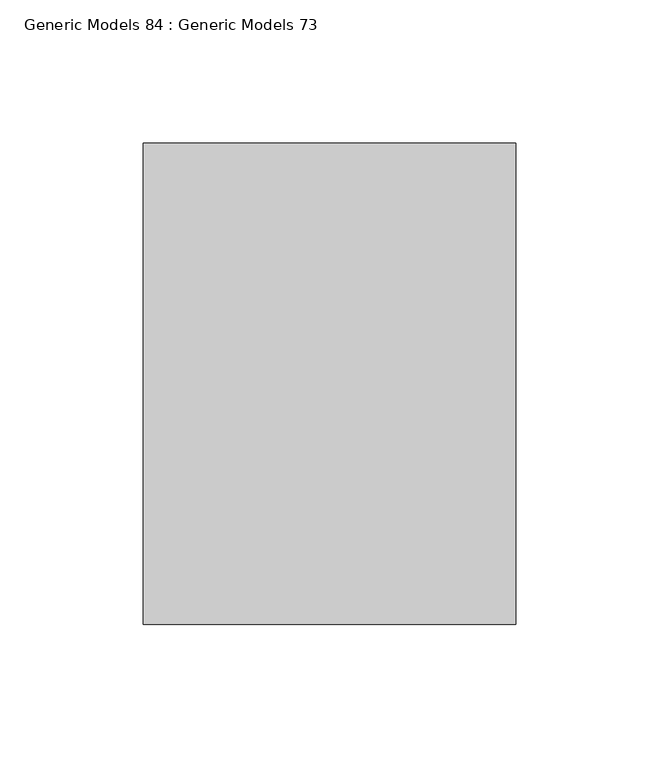
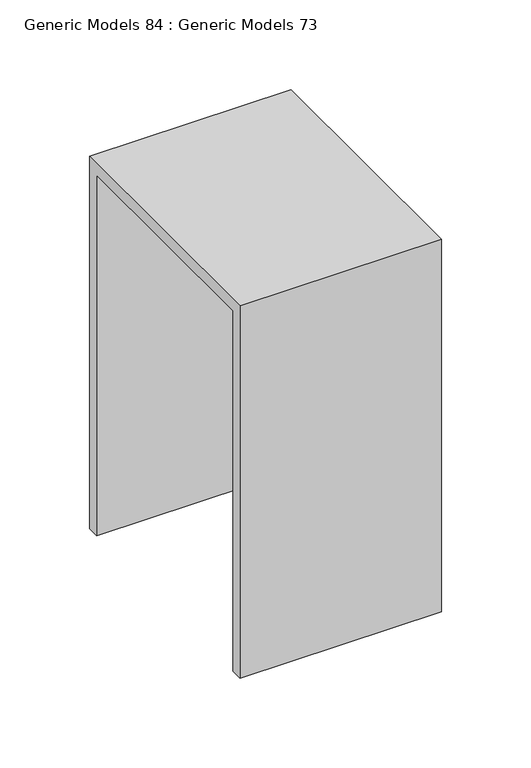
"""IFC4 building model written with IfcOpenShell, lengths in millimetres: proxy geometry, Generic Models 84 : Generic Models 73."""

from ifc_helpers import new_model, si_unit, frame, origin, place, context, project, spatial, polyline, outline, extrude, source, transform, mapped, element, save


def generic_models_84_generic_models_73_a949b104(model_context):
    return source(origin(), model_context, "Body", "SweptSolid", [
        extrude(outline(polyline([(36483.6207942, 271462.5), (36331.2207942, 271462.5), (36331.2207942, 271216.4375), (36323.2832942, 271216.4375), (36323.2832942, 271470.4375), (36491.5582942, 271470.4375), (36491.5582942, 271216.4375), (36483.6207942, 271216.4375), (36483.6207942, 271462.5)])), frame((31910.3221032, 0.0, 0.0), z_axis=(1.0, 0.0, 0.0), x_axis=(0.0, 1.0, 0.0)), (0.0, 0.0, 1.0), 130.175),
    ])


if __name__ == "__main__":
    model = new_model("IFC4")
    model_context = context("Model", 3, world=origin())
    ifc_project = project(units=[si_unit("LENGTHUNIT", "METRE", prefix="MILLI")], contexts=[model_context])
    site = spatial("IfcSite", under=ifc_project)
    building = spatial("IfcBuilding", under=site)
    placement = place(None, origin())
    generic_models_84_generic_models_73_shape = generic_models_84_generic_models_73_a949b104(model_context)
    element("IfcBuildingElementProxy", 1, Name="Generic Models 84 : Generic Models 73", ObjectType="Generic Models 84 : Generic Models 73", at=placement, inside=building, context=model_context, shape_type="MappedRepresentation", body=[
        mapped(generic_models_84_generic_models_73_shape, transform((0.0, 0.0, 0.0), x_axis=(1.0, 0.0, 0.0), y_axis=(0.0, 1.0, 0.0), z_axis=(0.0, 0.0, 1.0))),
    ])
    save(model, "model.ifc")

# Revit data of these elements
# Element 1 (IfcBuildingElementProxy, "Generic Models 84 : Generic Models 73")
#   Materials on its faces: "5/16 x5\" BENT PLATE CAP \nW/ 2 1\"DIA. THRU BOLTS"
# Materials
#   "5/16 x5\" BENT PLATE CAP \nW/ 2 1\"DIA. THRU BOLTS": class "Metal", colour RGB 199 199 199, transparency 0, Description = "Carbon steel", Cost = 0
